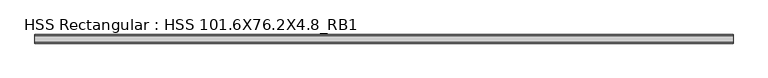
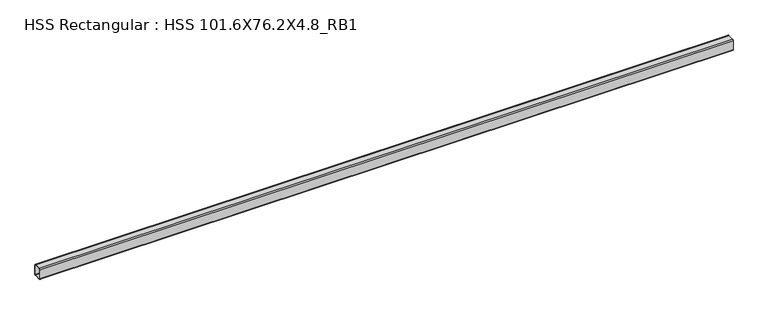
"""IFC4 building model written with IfcOpenShell, lengths in millimetres: beam geometry, HSS Rectangular : HSS 101.6X76.2X4.8_RB1."""

from ifc_helpers import new_model, si_unit, point, frame, frame_2d, origin, place, context, project, spatial, polyline, circle_curve, trimmed, segment, composite_curve, outline, extrude, source, transform, mapped, element, save


def hss_rectangular_hss_101_6x76_2x4_8_rb1_d08ab85d(model_context):
    return source(origin(), model_context, "Body", "SweptSolid", [
        extrude(outline(composite_curve([segment(polyline([(38.1, 41.275), (38.1, -41.275)]), True, "CONTINUOUS"), segment(trimmed(circle_curve(frame_2d((28.575, -41.275)), 9.525), [point((38.1, -41.275))], [point((28.575, -50.8))], False, "CARTESIAN"), True, "CONTINUOUS"), segment(polyline([(28.575, -50.8), (-28.575, -50.8)]), True, "CONTINUOUS"), segment(trimmed(circle_curve(frame_2d((-28.575, -41.275)), 9.525), [point((-28.575, -50.8))], [point((-38.1, -41.275))], False, "CARTESIAN"), True, "CONTINUOUS"), segment(polyline([(-38.1, -41.275), (-38.1, 41.275)]), True, "CONTINUOUS"), segment(trimmed(circle_curve(frame_2d((-28.575, 41.275)), 9.525), [point((-38.1, 41.275))], [point((-28.575, 50.8))], False, "CARTESIAN"), True, "CONTINUOUS"), segment(polyline([(-28.575, 50.8), (28.575, 50.8)]), True, "CONTINUOUS"), segment(trimmed(circle_curve(frame_2d((28.575, 41.275)), 9.525), [point((28.575, 50.8))], [point((38.1, 41.275))], False, "CARTESIAN"), True, "CONTINUOUS")], self_intersect=False), holes=[composite_curve([segment(trimmed(circle_curve(frame_2d((-28.575, 41.275)), 4.7625), [point((-28.575, 46.0375))], [point((-33.3375, 41.275))], True, "CARTESIAN"), True, "CONTINUOUS"), segment(polyline([(-33.3375, 41.275), (-33.3375, -41.275)]), True, "CONTINUOUS"), segment(trimmed(circle_curve(frame_2d((-28.575, -41.275)), 4.7625), [point((-33.3375, -41.275))], [point((-28.575, -46.0375))], True, "CARTESIAN"), True, "CONTINUOUS"), segment(polyline([(-28.575, -46.0375), (28.575, -46.0375)]), True, "CONTINUOUS"), segment(trimmed(circle_curve(frame_2d((28.575, -41.275)), 4.7625), [point((28.575, -46.0375))], [point((33.3375, -41.275))], True, "CARTESIAN"), True, "CONTINUOUS"), segment(polyline([(33.3375, -41.275), (33.3375, 41.275)]), True, "CONTINUOUS"), segment(trimmed(circle_curve(frame_2d((28.575, 41.275)), 4.7625), [point((33.3375, 41.275))], [point((28.575, 46.0375))], True, "CARTESIAN"), True, "CONTINUOUS"), segment(polyline([(28.575, 46.0375), (-28.575, 46.0375)]), True, "CONTINUOUS")], self_intersect=False)]), frame((-7610.9509957, 0.0, 0.0), z_axis=(1.0, 0.0, 0.0), x_axis=(0.0, 1.0, 0.0)), (0.0, 0.0, 1.0), 6134.9014192),
    ])


if __name__ == "__main__":
    model = new_model("IFC4")
    model_context = context("Model", 3, world=origin())
    ifc_project = project(units=[si_unit("LENGTHUNIT", "METRE", prefix="MILLI")], contexts=[model_context])
    site = spatial("IfcSite", under=ifc_project)
    building = spatial("IfcBuilding", under=site)
    placement = place(None, origin())
    hss_rectangular_hss_101_6x76_2x4_8_rb1_shape = hss_rectangular_hss_101_6x76_2x4_8_rb1_d08ab85d(model_context)
    element("IfcBeam", 1, ObjectType="HSS Rectangular : HSS 101.6X76.2X4.8_RB1", at=placement, inside=building, context=model_context, shape_type="MappedRepresentation", body=[
        mapped(hss_rectangular_hss_101_6x76_2x4_8_rb1_shape, transform((0.0, 0.0, 0.0), x_axis=(1.0, 0.0, 0.0), y_axis=(0.0, 1.0, 0.0), z_axis=(0.0, 0.0, 1.0))),
    ])
    save(model, "model.ifc")

# Revit data of these elements
# Type "HSS Rectangular : HSS 101.6X76.2X4.8_RB1"
#   Section Name Key = "HSS 4X3X3/16"
#   Assembly Code = "B10"
#   Width = 7.62 cm
#   Wall Nominal Thickness = 0.4763 cm
#   Wall Design Thickness = 0.442 cm
#   Torsional Moment of Inertia = 260.561 cm⁴
#   Torsional Modulus = 61.2876 cm³
#   Section Area = 14.4516 cm²
#   Plastic Modulus weak axis = 40.3122 cm³
#   Plastic Modulus strong axis = 49.1612 cm³
#   Perimeter = 0.881482 m²/m
#   Outer Fillet = 0.9525 cm
#   Nominal Weight = 12.1285 kgf/m
#   Moment of Inertia weak axis = 131.529 cm⁴
#   Moment of Inertia strong axis = 205.202 cm⁴
#   Inner Fillet = 0.4763 cm
#   Height = 10.16 cm
#   Elastic Modulus weak axis = 34.4128 cm³
#   Elastic Modulus strong axis = 40.476 cm³
#   Centroid Vertical = 5.08 cm
#   Centroid Horizontal = 3.81 cm
#   Length [instance default] = 1524 mm
#   Structural Material [instance default] = Steel ASTM A500, Grade B, Rectangular and Square
#   Principal Axes Angle = 0
# Element 1 (IfcBeam, "HSS Rectangular : HSS 101.6X76.2X4.8_RB1")
#   Structural Material = Steel ASTM A992
#   Materials on its faces: "Steel ASTM A992"
# Materials
#   "Steel ASTM A500, Grade B, Rectangular and Square": class "Metal", colour RGB 199 199 199, transparency 0, Description = "Carbon steel", Cost = 0
#   "Steel ASTM A992": class "Metal", colour RGB 199 199 199, transparency 0, Description = "Structural steel 50ksi", Cost = 0
